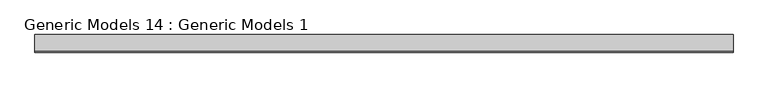
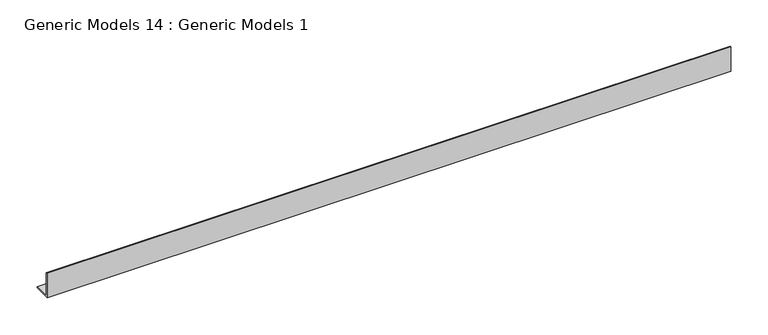
"""IFC4 building model written with IfcOpenShell, lengths in millimetres: proxy geometry, Generic Models 14 : Generic Models 1."""

from ifc_helpers import new_model, si_unit, frame, origin, place, context, project, spatial, polyline, outline, extrude, source, transform, mapped, element, save


def generic_models_14_generic_models_1_67ce90fe(model_context):
    return source(origin(), model_context, "Body", "SweptSolid", [
        extrude(outline(polyline([(39604.1428995, 2654.3), (39605.7303995, 2654.3), (39605.7303995, 2616.2), (39631.1303995, 2616.2), (39631.1303995, 2614.6125), (39604.1428995, 2614.6125), (39604.1428995, 2654.3)])), frame((51512.0577305, 0.0, 0.0), z_axis=(1.0, 0.0, 0.0), x_axis=(0.0, 1.0, 0.0)), (0.0, 0.0, 1.0), 1066.8),
    ])


if __name__ == "__main__":
    model = new_model("IFC4")
    model_context = context("Model", 3, world=origin())
    ifc_project = project(units=[si_unit("LENGTHUNIT", "METRE", prefix="MILLI")], contexts=[model_context])
    site = spatial("IfcSite", under=ifc_project)
    building = spatial("IfcBuilding", under=site)
    placement = place(None, origin())
    generic_models_14_generic_models_1_shape = generic_models_14_generic_models_1_67ce90fe(model_context)
    element("IfcBuildingElementProxy", 1, Name="Generic Models 14 : Generic Models 1", ObjectType="Generic Models 14 : Generic Models 1", at=placement, inside=building, context=model_context, shape_type="MappedRepresentation", body=[
        mapped(generic_models_14_generic_models_1_shape, transform((0.0, 0.0, 0.0), x_axis=(1.0, 0.0, 0.0), y_axis=(0.0, 1.0, 0.0), z_axis=(0.0, 0.0, 1.0))),
    ])
    save(model, "model.ifc")

# Revit data of these elements
# Element 1 (IfcBuildingElementProxy, "Generic Models 14 : Generic Models 1")
#   Materials on its faces: "ACOUSTICAL PERMITER TRACK TO MATCH EXISTING"
# Materials
#   "ACOUSTICAL PERMITER TRACK TO MATCH EXISTING": class "Generic", colour RGB 120 120 120, transparency 0, Cost = 0
